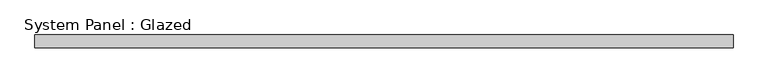
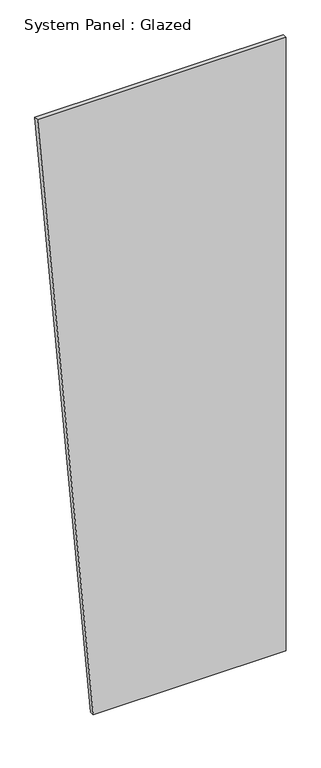
"""IFC4 building model written with IfcOpenShell, lengths in millimetres: plate geometry, System Panel : Glazed."""

from ifc_helpers import new_model, si_unit, frame, origin, place, context, project, spatial, polyline, outline, extrude, source, transform, mapped, element, save


def system_panel_glazed_cde5e94a(model_context):
    return source(origin(), model_context, "Body", "SweptSolid", [
        extrude(outline(polyline([(0.0, -386.1685195), (0.0, 701.3055584), (3657.6, 701.3055584), (3657.6, -701.3055584), (0.0, -386.1685195)])), frame((0.0, -44.45, 0.0), z_axis=(0.0, 1.0, 0.0), x_axis=(0.0, 0.0, 1.0)), (0.0, 0.0, 1.0), 25.4),
    ])


if __name__ == "__main__":
    model = new_model("IFC4")
    model_context = context("Model", 3, world=origin())
    ifc_project = project(units=[si_unit("LENGTHUNIT", "METRE", prefix="MILLI")], contexts=[model_context])
    site = spatial("IfcSite", under=ifc_project)
    building = spatial("IfcBuilding", under=site)
    placement = place(None, origin())
    system_panel_glazed_shape = system_panel_glazed_cde5e94a(model_context)
    element("IfcPlate", 1, ObjectType="System Panel : Glazed", at=placement, inside=building, context=model_context, shape_type="MappedRepresentation", body=[
        mapped(system_panel_glazed_shape, transform((0.0, 0.0, 0.0), x_axis=(1.0, 0.0, 0.0), y_axis=(0.0, 1.0, 0.0), z_axis=(0.0, 0.0, 1.0))),
    ])
    save(model, "model.ifc")

# Revit data of these elements
# Type "System Panel : Glazed"
#   Construction Type Id = "GSP4R"
#   Analytic Construction = "1/8 in Pilkington single glazing"
#   Visual Light Transmittance = 0.9
#   Solar Heat Gain Coefficient = 0.86
#   Heat Transfer Coefficient (U) = 1.18115 BTU/(h·ft²·°F)
#   Define Thermal Properties by = 1
# Element 1 (IfcPlate, "System Panel : Glazed")
#   Materials on its faces: "Glass"
# Materials
#   "Glass": class "Glass", colour RGB 0 128 192, transparency 0.75, Description = "Soda Lime Glass", Cost = 0
